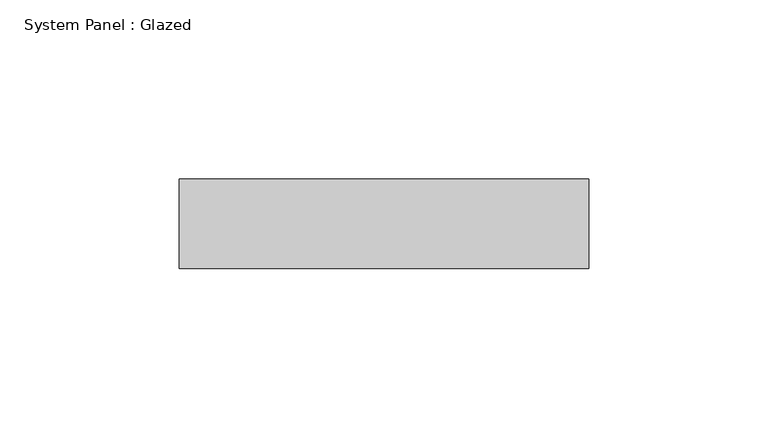
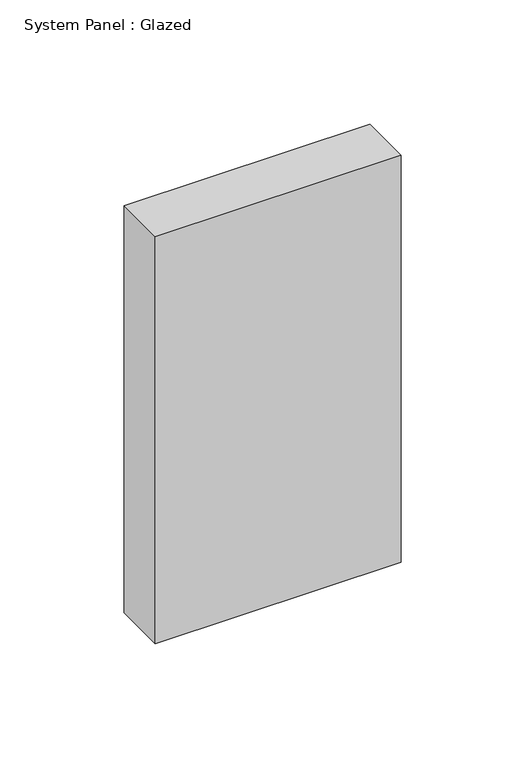
"""IFC4 building model written with IfcOpenShell, lengths in millimetres: plate geometry, System Panel : Glazed."""

from ifc_helpers import new_model, si_unit, origin, origin_with_axes, place, context, project, spatial, polyline, outline, extrude, source, transform, mapped, element, save


def system_panel_glazed_41e93d41(model_context):
    return source(origin(), model_context, "Body", "SweptSolid", [
        extrude(outline(polyline([(57.080979, 24.5), (-57.080979, 24.5), (-57.080979, 49.5), (57.080979, 49.5), (57.080979, 24.5)])), origin_with_axes(), (0.0, 0.0, 1.0), 200.0),
    ])


if __name__ == "__main__":
    model = new_model("IFC4")
    model_context = context("Model", 3, world=origin())
    ifc_project = project(units=[si_unit("LENGTHUNIT", "METRE", prefix="MILLI")], contexts=[model_context])
    site = spatial("IfcSite", under=ifc_project)
    building = spatial("IfcBuilding", under=site)
    placement = place(None, origin())
    system_panel_glazed_shape = system_panel_glazed_41e93d41(model_context)
    element("IfcPlate", 1, ObjectType="System Panel : Glazed", at=placement, inside=building, context=model_context, shape_type="MappedRepresentation", body=[
        mapped(system_panel_glazed_shape, transform((0.0, 0.0, 0.0), x_axis=(1.0, 0.0, 0.0), y_axis=(0.0, 1.0, 0.0), z_axis=(0.0, 0.0, 1.0))),
    ])
    save(model, "model.ifc")

# Revit data of these elements
# Element 1 (IfcPlate, "System Panel : Glazed")
#   Materials on its faces: "Glass"
# Materials
#   "Glass": class "Glass", colour RGB 218 227 224, transparency 0.85, Description = "Soda Lime Glass", Cost = 0
